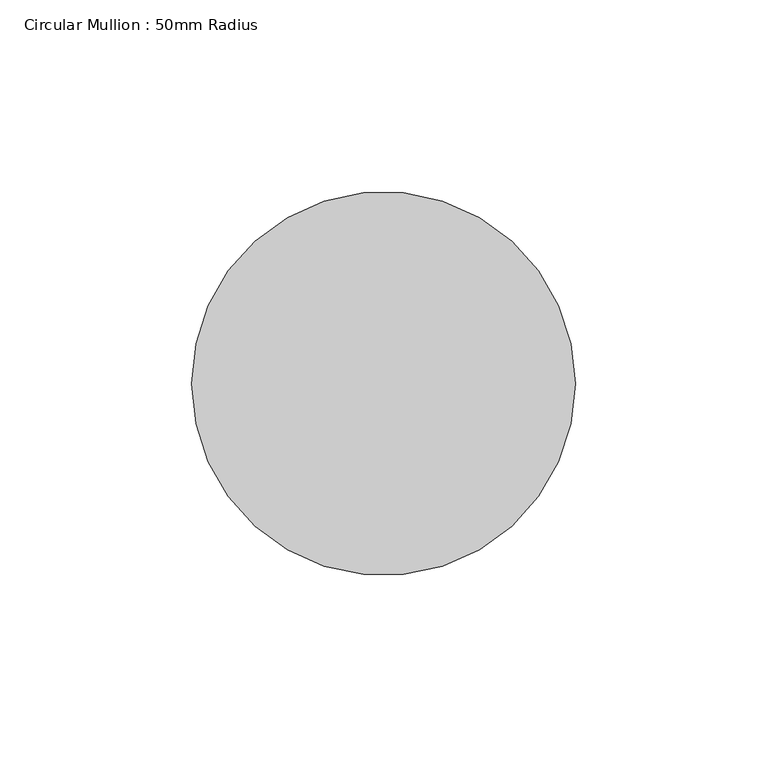
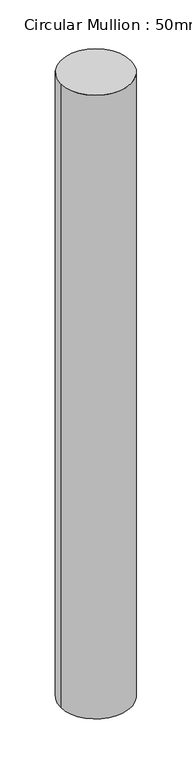
"""IFC4 building model written with IfcOpenShell, lengths in millimetres: member geometry, Circular Mullion : 50mm Radius."""

from ifc_helpers import new_model, si_unit, point, frame, origin, origin_2d, place, context, project, spatial, circle_curve, trimmed, segment, composite_curve, outline, extrude, source, transform, mapped, element, save


def circular_mullion_50mm_radius_95b071aa(model_context):
    return source(origin(), model_context, "Body", "SweptSolid", [
        extrude(outline(composite_curve([segment(trimmed(circle_curve(origin_2d(), 50.0), [point((50.0, 0.0))], [point((-50.0, 0.0))], False, "CARTESIAN"), True, "CONTINUOUS"), segment(trimmed(circle_curve(origin_2d(), 50.0), [point((-50.0, 0.0))], [point((50.0, 0.0))], False, "CARTESIAN"), True, "CONTINUOUS")], self_intersect=False)), frame((0.0, 0.0, -940.2191858), z_axis=(0.0, 0.0, 1.0), x_axis=(1.0, 0.0, 0.0)), (0.0, 0.0, 1.0), 940.2191858),
    ])


if __name__ == "__main__":
    model = new_model("IFC4")
    model_context = context("Model", 3, world=origin())
    ifc_project = project(units=[si_unit("LENGTHUNIT", "METRE", prefix="MILLI")], contexts=[model_context])
    site = spatial("IfcSite", under=ifc_project)
    building = spatial("IfcBuilding", under=site)
    placement = place(None, origin())
    circular_mullion_50mm_radius_shape = circular_mullion_50mm_radius_95b071aa(model_context)
    element("IfcMember", 1, ObjectType="Circular Mullion : 50mm Radius", at=placement, inside=building, context=model_context, shape_type="MappedRepresentation", body=[
        mapped(circular_mullion_50mm_radius_shape, transform((0.0, 0.0, 0.0), x_axis=(1.0, 0.0, 0.0), y_axis=(0.0, 1.0, 0.0), z_axis=(0.0, 0.0, 1.0))),
    ])
    save(model, "model.ifc")

# Revit data of these elements
# Type "Circular Mullion : 50mm Radius"
#   built-in parameter 1007350 = 0.164042 (stored number, unit not read)
# Element 1 (IfcMember, "Circular Mullion : 50mm Radius")
#   Materials on its faces: "Aluminium"
# Materials
#   "Aluminium": class "Metal", colour RGB 247 247 247, transparency 0, Description = "Aluminium 6061", Cost = 0
